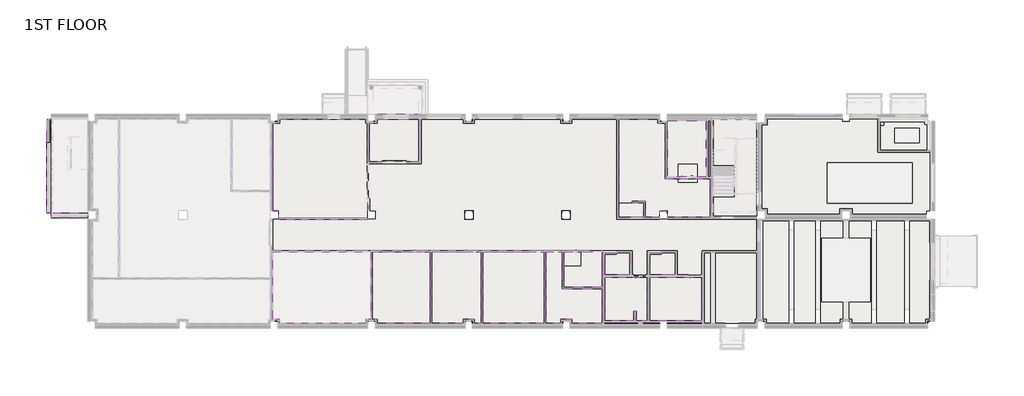
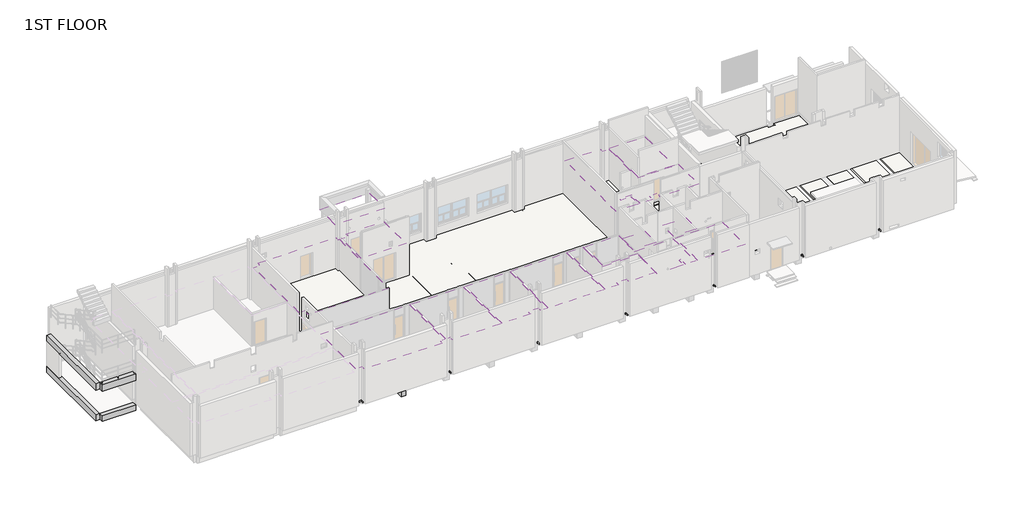
# One storey, part 8 of 15: 26 slabs, 15 coverings, 5 beams.
# Revit data of these elements (continued)
# Type "H_CE_AR_B09_2L Gypsum Board_T Bar_9T_C4" (continued)
#   Layers, outside or top first: 9.5 mm "00_Finish_Gypsum Board" (function 4); 9.5 mm "00_Finish_Gypsum Board" (function 4)
# Type "H_CE_AR_B09_Aluminum Spandrel_M Bar_0.8T_C9"
#   built-in parameter 1002203 = 1 (stored number, unit not read)
#   built-in parameter 1002202 = 1 (stored number, unit not read)
#   Layers, outside or top first: 0.8 mm "00.Ceiling_Aluminum Spandrel" (function 4)
# Type "H_CE_AR_B09_SMC Ceiling_T Bar_300x300x0.8T_C6"
#   built-in parameter 1002203 = 1 (stored number, unit not read)
#   built-in parameter 1002202 = 1 (stored number, unit not read)
#   Layers, outside or top first: 0.8 mm "00.Ceiling_SMC" (function 4)
# Type "H_CE_AR_B09_Souns Absorbing Soft Fiber Board_T Bar_600x600x9T_C5"
#   built-in parameter 1002203 = 1 (stored number, unit not read)
#   built-in parameter 1002202 = 1 (stored number, unit not read)
#   Layers, outside or top first: 9 mm "00.Ceiling_Sound Absorbing Soft Fiber Board" (function 4)
# Type "H_CE_AR_B09_Stainless Hairline Finish_3T"
#   built-in parameter 1002203 = 1 (stored number, unit not read)
#   built-in parameter 1002202 = 1 (stored number, unit not read)
#   Layers, outside or top first: 3 mm "00.Finish_Stainless Hairline" (function 4)
# Type "H_FL_AR_S17_RC Slab_T150_1S1"
#   Keynote = ""
#   Type Comments = "CV-AG"
#   Description = ""
#   H_Rebar Ratio = 0.1
#   Function = 1
#   Layers, outside or top first: 150 mm "Concrete_f'c=28MPa(Cylender)" (function 1)
# Type "H_FL_AR_S17_RC Slab_T150_GS1"
#   Keynote = ""
#   Type Comments = "CV-AG"
#   Description = ""
#   H_Rebar Ratio = 0.1
#   Function = 1
#   Layers, outside or top first: 150 mm "Concrete_f'c=28MPa(Cylender)" (function 1)
# Type "H_FL_AR_S17_RC Slab_T200_SS1"
#   Keynote = ""
#   Type Comments = "CV-AG"
#   Description = ""
#   H_Rebar Ratio = 0.1
#   Function = 1
#   Layers, outside or top first: 200 mm "Concrete_f'c=28MPa(Cylender)" (function 1)
# Type "H_FL_AR_B07_Wood Tile_600x600xT3_F8"
#   Keynote = ""
#   Type Comments = "Finish"
#   Description = ""
#   Function = 1
#   Layers, outside or top first: 3 mm "00_Finish_Wood Tile" (function 4); 27 mm "00_Concrete_Cement Mortar" (function 1)
# Type "H_FL_AR_B07_Deco Tile_600x600xT3"
#   Keynote = ""
#   Type Comments = "Finish"
#   Description = ""
#   Function = 1
#   Layers, outside or top first: 3 mm "00_Finish_Deco Tile" (function 4); 27 mm "00_Concrete_Cement Mortar" (function 1)
# Type "H_FL_AR_B07_Polishing Tile_600x600xT3"
#   Keynote = ""
#   Type Comments = "Finish"
#   Description = ""
#   Function = 1
#   Layers, outside or top first: 3 mm "00_Finish_Polishing Tile" (function 4); 27 mm "00_Concrete_Cement Mortar" (function 1)
# Type "H_FL_AR_B07_Capet Tile_600x600xT3"
#   Keynote = ""
#   Type Comments = "Finish"
#   Description = ""
#   Function = 1
#   Layers, outside or top first: 3 mm "00_Finish_Carpet Tile" (function 4); 27 mm "00_Concrete_Cement Mortar" (function 1)
# Type "H_FL_AR_B07_Wood Tile_600x600xT110_F8"
#   Keynote = ""
#   Type Comments = "Finish"
#   Description = ""
#   Function = 1
#   Layers, outside or top first: 3 mm "00_Finish_Wood Tile" (function 4); 107 mm "00_Concrete_Cement Mortar" (function 1)
# Type "H_FL_AR_B07_Non-Slip Ceramic Tile_L Waterproof_300x300xT4"
#   Keynote = ""
#   Type Comments = "Finish"
#   Description = ""
#   Function = 0
#   Layers, outside or top first: 4 mm "00_Finish_Ceramic Tile" (function 4); 96 mm "00_Concrete_Cement Mortar" (function 1)
# Type "H_FL_AR_B07_Granite Tile_150x150xT30"
#   Keynote = ""
#   Type Comments = "Finish"
#   Description = ""
#   Function = 0
#   Layers, outside or top first: 30 mm "00_Stone_Granite" (function 4); 60 mm "00_Concrete_Cement Mortar" (function 1)
# Type "H_FL_AR_B07_Granite Tile_150x150xT30(Mortar_T170)"
#   Keynote = ""
#   Type Comments = "Finish"
#   Description = ""
#   Function = 0
#   Layers, outside or top first: 30 mm "00_Stone_Granite" (function 4); 170 mm "00_Concrete_Cement Mortar" (function 1)
# Type "H_FL_AR_S17_RC Slab_T300"
#   Keynote = ""
#   Type Comments = "CV-AG"
#   Description = ""
#   H_Rebar Ratio = 0.12
#   Function = 1
#   Layers, outside or top first: 300 mm "Concrete_f'c=28MPa(Cylender)" (function 1)
# Element 1 (IfcBeam, "RC Beam_Rectangular : H_SB_AR S16_TG-UG_450x800_1B1A")
#   Comments = ""
#   hec_material3 = none
#   hec_material2 = none
#   hec_material1 = none
#   Structural Material = Concrete_f'c=28MPa(Cylender)
#   Phase Created = New Construction
#   Materials on its faces: "Concrete_f'c=28MPa(Cylender)"
# Element 2 (IfcBeam, "RC Beam_Rectangular : H_SB_AR S16_RC Beam-AG_400x530_SG1A")
#   Comments = ""
#   hec_material3 = none
#   hec_material2 = none
#   hec_material1 = none
#   Structural Material = Concrete_f'c=28MPa(Cylender)
#   Phase Created = New Construction
#   Materials on its faces: "Concrete_f'c=28MPa(Cylender)"
# Element 3 (IfcBeam, "RC Beam_Rectangular : H_SB_AR S16_RC Beam-AG_400x600_SG2")
#   Comments = ""
#   hec_material3 = none
#   hec_material2 = none
#   hec_material1 = none
#   Structural Material = Concrete_f'c=28MPa(Cylender)
#   Phase Created = New Construction
#   Materials on its faces: "Concrete_f'c=28MPa(Cylender)"
# Element 4 (IfcBeam, "RC Beam_Rectangular : H_SB_AR S16_RC Beam-AG_400x600_SWG2")
#   Comments = ""
#   hec_material3 = none
#   hec_material2 = none
#   hec_material1 = none
#   Structural Material = Concrete_f'c=28MPa(Cylender)
#   Phase Created = New Construction
#   Materials on its faces: "Concrete_f'c=28MPa(Cylender)"
# Element 5 (IfcBeam, "RC Beam_Rectangular : H_SB_AR S16_RC Beam-AG_400x600_SG1")
#   Comments = ""
#   hec_material3 = none
#   hec_material2 = none
#   hec_material1 = none
#   Structural Material = Concrete_f'c=28MPa(Cylender)
#   Phase Created = New Construction
#   Materials on its faces: "Concrete_f'c=28MPa(Cylender)"
# Elements 6, 10, 11, 13 (IfcCovering, "H_CE_AR_B09_2L Gypsum Board_T Bar_9T_C4")
#   Height Offset From Level = 3030 mm
#   Phase Created = New Construction
#   Materials on its faces: "00_Finish_Gypsum Board"
# Element 7 (IfcCovering, "H_CE_AR_B09_Aluminum Spandrel_M Bar_0.8T_C9")
#   Height Offset From Level = 3030 mm
#   Phase Created = New Construction
#   Materials on its faces: "00.Ceiling_Aluminum Spandrel"
# Element 8 (IfcCovering, "H_CE_AR_B09_2L Gypsum Board_T Bar_9T_C4")
#   Height Offset From Level = 3110 mm
#   Phase Created = New Construction
#   Materials on its faces: "00_Finish_Gypsum Board"
# Element 9 (IfcCovering, "H_CE_AR_B09_SMC Ceiling_T Bar_300x300x0.8T_C6")
#   Height Offset From Level = 3000 mm
#   Phase Created = New Construction
#   Materials on its faces: "00.Ceiling_SMC"
# Elements 12, 14, 15 (IfcCovering, "H_CE_AR_B09_Souns Absorbing Soft Fiber Board_T Bar_600x600x9T_C5")
#   Height Offset From Level = 3030 mm
#   Phase Created = New Construction
#   Materials on its faces: "00.Ceiling_Sound Absorbing Soft Fiber Board"
# Elements 16, 17, 18, 19 (IfcCovering, "H_CE_AR_B09_2L Gypsum Board_T Bar_9T_C4")
#   Height Offset From Level = 2700 mm
#   Phase Created = New Construction
#   Materials on its faces: "00_Finish_Gypsum Board"
# Element 20 (IfcCovering, "H_CE_AR_B09_Stainless Hairline Finish_3T")
#   Height Offset From Level = 3900 mm
#   Phase Created = New Construction
#   Materials on its faces: "00.Finish_Stainless Hairline"
# Element 21 (IfcSlab, "H_FL_AR_S17_RC Slab_T150_1S1")
#   Comments = ""
#   TMP_Element Name = "SS2"
#   Height Offset From Level = 0 mm
#   built-in parameter 1001954 = 1
#   Phase Created = New Construction
#   Materials on its faces: "Concrete_f'c=28MPa(Cylender)"
# Element 22 (IfcSlab, "H_FL_AR_S17_RC Slab_T150_1S1")
#   Comments = ""
#   TMP_Element Name = "SS2"
#   Height Offset From Level = -100 mm
#   built-in parameter 1001954 = 1
#   Phase Created = New Construction
#   Materials on its faces: "Concrete_f'c=28MPa(Cylender)"
# Element 23 (IfcSlab, "H_FL_AR_S17_RC Slab_T150_GS1")
#   Comments = ""
#   TMP_Element Name = "SS2"
#   built-in parameter 1001955 = 3.14159 (stored number, unit not read)
#   Height Offset From Level = 0 mm
#   built-in parameter 1001954 = 1
#   Phase Created = New Construction
#   Materials on its faces: "Concrete_f'c=28MPa(Cylender)"
# Element 24 (IfcSlab, "H_FL_AR_S17_RC Slab_T150_1S1")
#   Comments = ""
#   TMP_Element Name = "SS2"
#   built-in parameter 1001955 = 3.14159 (stored number, unit not read)
#   Height Offset From Level = -100 mm
#   built-in parameter 1001954 = 1
#   Phase Created = New Construction
#   Materials on its faces: "Concrete_f'c=28MPa(Cylender)"
# Element 25 (IfcSlab, "H_FL_AR_S17_RC Slab_T200_SS1")
#   Comments = ""
#   TMP_Element Name = "SS2"
#   Height Offset From Level = 0 mm
#   built-in parameter 1001954 = 1
#   Phase Created = New Construction
#   Materials on its faces: "Concrete_f'c=28MPa(Cylender)"
# Element 26 (IfcSlab, "H_FL_AR_S17_RC Slab_T150_GS1")
#   Comments = ""
#   TMP_Element Name = "SS2"
#   Height Offset From Level = 0 mm
#   built-in parameter 1001954 = 1
#   Phase Created = New Construction
#   Materials on its faces: "Concrete_f'c=28MPa(Cylender)"
# Elements 27, 43 (IfcSlab, "H_FL_AR_B07_Wood Tile_600x600xT3_F8")
#   Height Offset From Level = 30 mm
#   Phase Created = New Construction
#   Materials on its faces: "00_Concrete_Cement Mortar", "00_Finish_Wood Tile"
# Elements 28, 31, 40, 42 (IfcSlab, "H_FL_AR_B07_Deco Tile_600x600xT3")
#   Height Offset From Level = 30 mm
#   Phase Created = New Construction
#   Materials on its faces: "00_Concrete_Cement Mortar", "00_Finish_Deco Tile"
# Element 29 (IfcSlab, "H_FL_AR_B07_Polishing Tile_600x600xT3")
#   built-in parameter 1001955 = 1.5708 (stored number, unit not read)
#   Height Offset From Level = 30 mm
#   Phase Created = New Construction
#   Materials on its faces: "00_Concrete_Cement Mortar", "00_Finish_Polishing Tile"
# Element 30 (IfcSlab, "H_FL_AR_B07_Wood Tile_600x600xT3_F8")
#   built-in parameter 1001955 = 1.5708 (stored number, unit not read)
#   Height Offset From Level = 30 mm
#   Phase Created = New Construction
#   Materials on its faces: "00_Concrete_Cement Mortar", "00_Finish_Wood Tile"
# Element 32 (IfcSlab, "H_FL_AR_B07_Capet Tile_600x600xT3")
#   Height Offset From Level = 30 mm
#   Phase Created = New Construction
#   Materials on its faces: "00_Concrete_Cement Mortar", "00_Finish_Carpet Tile"
# Element 33 (IfcSlab, "H_FL_AR_B07_Deco Tile_600x600xT3")
#   built-in parameter 1001955 = 1.5708 (stored number, unit not read)
#   Height Offset From Level = 30 mm
#   Phase Created = New Construction
#   Materials on its faces: "00_Concrete_Cement Mortar", "00_Finish_Deco Tile"
# Element 34 (IfcSlab, "H_FL_AR_B07_Wood Tile_600x600xT110_F8")
#   Height Offset From Level = 110 mm
#   Phase Created = New Construction
#   Materials on its faces: "00_Concrete_Cement Mortar", "00_Finish_Wood Tile"
# Elements 35, 36, 37, 38, 41 (IfcSlab, "H_FL_AR_B07_Non-Slip Ceramic Tile_L Waterproof_300x300xT4")
#   Height Offset From Level = 0 mm
#   Phase Created = New Construction
#   Materials on its faces: "00_Concrete_Cement Mortar", "00_Finish_Ceramic Tile"
# Element 39 (IfcSlab, "H_FL_AR_B07_Wood Tile_600x600xT110_F8")
#   built-in parameter 1001955 = 1.5708 (stored number, unit not read)
#   Height Offset From Level = 110 mm
#   Phase Created = New Construction
#   Materials on its faces: "00_Concrete_Cement Mortar", "00_Finish_Wood Tile"
# Element 44 (IfcSlab, "H_FL_AR_B07_Granite Tile_150x150xT30")
#   Height Offset From Level = 200 mm
#   Phase Created = New Construction
#   Materials on its faces: "00_Concrete_Cement Mortar", "00_Stone_Granite"
# Element 45 (IfcSlab, "H_FL_AR_B07_Granite Tile_150x150xT30(Mortar_T170)")
#   Height Offset From Level = 200 mm
#   Phase Created = New Construction
#   Materials on its faces: "00_Concrete_Cement Mortar", "00_Stone_Granite"
# Element 46 (IfcSlab, "H_FL_AR_S17_RC Slab_T300")
#   Comments = ""
#   TMP_Element Name = "SS2"
#   Height Offset From Level = -150 mm
#   built-in parameter 1001954 = 1
#   Phase Created = New Construction
#   Materials on its faces: "Concrete_f'c=28MPa(Cylender)"
# Materials
#   "00_Finish_Gypsum Board": class "Finish", colour RGB 171 170 168, transparency 0, Description = "Gypsum Board", Cost = 0, Image = Finishes.Gypsum Board.Painted.White.jpg
#   "00.Ceiling_Aluminum Spandrel": class "Generic", colour RGB 253 254 255, transparency 0, Description = "Acoustic ceiling tile", Cost = 0
#   "00.Ceiling_SMC": class "Generic", colour RGB 237 237 236, transparency 0, Description = "Acoustic ceiling tile", Cost = 0
#   "00.Ceiling_Sound Absorbing Soft Fiber Board": class "Generic", colour RGB 237 237 236, transparency 0, Description = "Acoustic ceiling tile", Cost = 0
#   "00.Finish_Stainless Hairline": class "Generic", colour RGB 149 149 149, transparency 0, Description = "Acoustic ceiling tile", Cost = 0
#   "Concrete_f'c=28MPa(Cylender)": class "Concrete", colour RGB 176 176 176, transparency 0, Description = "Reinf. Conc.", Cost = 0, Image = Concrete.Cast-In-Place.Flat.Polished.Grey.jpg
#   "00_Finish_Wood Tile": class "Finish", colour RGB 233 219 207, transparency 0, Description = "Ceramic Tile", Cost = 0
#   "00_Concrete_Cement Mortar": class "Concrete", colour RGB 183 186 184, transparency 0, Description = "Cement Mortar", Cost = 0, Image = Concrete.Cast-In-Place.Flat.Broom.Grey.jpg
#   "00_Finish_Deco Tile": class "Finish", colour RGB 245 245 245, transparency 0, Description = "Ceramic Tile", Cost = 0
#   "00_Finish_Polishing Tile": class "Finish", colour RGB 245 245 245, transparency 0, Description = "Ceramic Tile", Cost = 0
#   "00_Finish_Carpet Tile": class "Finish", colour RGB 68 67 66, transparency 0, Description = "Carpet", Cost = 0
#   "00_Finish_Ceramic Tile": class "Finish", colour RGB 245 245 245, transparency 0, Description = "Ceramic Tile", Cost = 0, Image = none
#   "00_Stone_Granite": class "Stone", colour RGB 99 103 98, transparency 0, Description = "Granite", Cost = 0, Image = Masonry.Stone.Granite.Square.Stacked.Polished.Black-White.jpg
# Room at (66747.5, -1477.5) mm, phase "New Construction", upper level "1ST FLOOR", upper offset 5800 mm, lower offset 0 mm
#   Comments = ""
#   Occupancy = "1"
#   Number = "124"
#   Name = "F.O TANK ROOM"
#   H_Room H or CH = 5.8 mm
# Room at (48912.5, -2537.5) mm, phase "New Construction", upper level "1ST FLOOR", upper offset 5800 mm, lower offset 0 mm
#   Comments = ""
#   Occupancy = "1"
#   Number = "109"
#   Name = "SHOWER ROOM"
#   H_Room H or CH = 3 mm
# Room at (61920.25, -12686.25) mm, phase "New Construction", upper level "1ST FLOOR", upper offset 5800 mm, lower offset 0 mm
#   Comments = ""
#   Occupancy = "1"
#   Number = "125"
#   Name = "HVAC ROOM"
#   H_Room H or CH = 5.8 mm
# Room at (24871.5, -1826.5) mm, phase "New Construction", upper level "1ST FLOOR", upper offset 5800 mm, lower offset 0 mm
#   Comments = ""
#   Occupancy = "1"
#   Number = "105"
#   Name = "AIR LOCK"
#   H_Room H or CH = 3 mm
# Room at (52496.5, -14023.5) mm, phase "New Construction", upper level "1ST FLOOR", upper offset 5800 mm, lower offset 0 mm
#   Comments = ""
#   Occupancy = "1"
#   Number = "122"
#   Name = "CYLINDER ROOM"
#   H_Room H or CH = 3 mm
# Room at (43200, -12000) mm, phase "New Construction", upper level "1ST FLOOR", upper offset 5800 mm, lower offset 0 mm
#   Comments = ""
#   Occupancy = "1"
#   Number = "118"
#   Name = "DISABLED TOLET(M)"
#   H_Room H or CH = 2.7 mm
# Room at (43900, -14887.5) mm, phase "New Construction", upper level "1ST FLOOR", upper offset 5800 mm, lower offset 0 mm
#   Comments = ""
#   Occupancy = "1"
#   Number = "120"
#   Name = "TOILET(M)"
#   H_Room H or CH = 2.7 mm
# Room at (46900, -12000) mm, phase "New Construction", upper level "1ST FLOOR", upper offset 5800 mm, lower offset 0 mm
#   Comments = ""
#   Occupancy = "1"
#   Number = "119"
#   Name = "DISABLED TOILET(W)"
#   H_Room H or CH = 2.7 mm
# Room at (48000, -14887.5) mm, phase "New Construction", upper level "1ST FLOOR", upper offset 5800 mm, lower offset 0 mm
#   Comments = ""
#   Occupancy = "1"
#   Number = "121"
#   Name = "TOILET(W)"
#   H_Room H or CH = 2.7 mm
# Room at (47084, -5635.02) mm, phase "New Construction", upper level "1ST FLOOR", upper offset 5800 mm, lower offset 0 mm
#   Comments = ""
#   Occupancy = "1"
#   Number = "108"
#   Name = "LOCKER ROOM"
#   H_Room H or CH = 3 mm
# Room at (34768, -8500) mm, phase "New Construction", upper level "1ST FLOOR", upper offset 5800 mm, lower offset 0 mm
#   Comments = ""
#   Occupancy = "1"
#   Number = "111"
#   Name = "CORRIDOR"
#   H_Room H or CH = 5.8 mm
# Room at (52862.5, -4131) mm, phase "New Construction", upper level "1ST FLOOR", upper offset 5800 mm, lower offset 0 mm
#   Comments = ""
#   Occupancy = "1"
#   Number = "110"
#   Name = "STAIRCASE"
#   H_Room H or CH = 5.8 mm
# Room at (62081, -3919) mm, phase "New Construction", upper level "1ST FLOOR", upper offset 9300 mm, lower offset 0 mm
#   Comments = ""
#   Number = "123"
#   Name = "EDG ROOM"
#   H_Room H or CH = 9.2 mm
# Room at (44419.201, -7539.972) mm, phase "New Construction", upper level "1ST FLOOR", upper offset 5800 mm, lower offset 0 mm
#   Comments = ""
#   Occupancy = "1"
#   Number = "151"
#   Name = "LOCKER ENTRANCE"
#   H_Room H or CH = 3 mm
# Room at (33678.344, -3773.505) mm, phase "New Construction", upper level "1ST FLOOR", upper offset 5800 mm, lower offset 0 mm
#   Comments = ""
#   Occupancy = "1"
#   Number = "107"
#   Name = "OFFICE ROOM"
#   H_Room H or CH = 5.8 mm
# Room at (40496.214, -12367.394) mm, phase "New Construction", upper level "1ST FLOOR", upper offset 5800 mm, lower offset 0 mm
#   Comments = ""
#   Occupancy = "1"
#   Number = "116"
#   Name = "MAMA'S REST ROOM"
#   H_Room H or CH = 3 mm
# Room at (39361.919, -14919.559) mm, phase "New Construction", upper level "1ST FLOOR", upper offset 5800 mm, lower offset 0 mm
#   Comments = ""
#   Occupancy = "1"
#   Number = "117"
#   Name = "STORAGE"
#   H_Room H or CH = 3 mm
# Room at (34862.546, -13898.693) mm, phase "New Construction", upper level "1ST FLOOR", upper offset 5800 mm, lower offset 0 mm
#   Comments = ""
#   Occupancy = "1"
#   Number = "115"
#   Name = "PRESIDENT ROOM"
#   H_Room H or CH = 3 mm
# Room at (30211.935, -13917.598) mm, phase "New Construction", upper level "1ST FLOOR", upper offset 5800 mm, lower offset 0 mm
#   Comments = ""
#   Occupancy = "1"
#   Number = "114"
#   Name = "PARTNER'S OFFICE"
#   H_Room H or CH = 3 mm
# Room at (25315.559, -14049.933) mm, phase "New Construction", upper level "1ST FLOOR", upper offset 5800 mm, lower offset 0 mm
#   Comments = ""
#   Occupancy = "1"
#   Number = "113"
#   Name = "REST ROOM"
#   H_Room H or CH = 3 mm
# Room at (19265.983, -13936.503) mm, phase "New Construction", upper level "1ST FLOOR", upper offset 5800 mm, lower offset 0 mm
#   Comments = ""
#   Occupancy = "1"
#   Number = "112"
#   Name = "CONFERENCE ROOM"
#   H_Room H or CH = 3 mm
# Room at (18995.787, -4264.529) mm, phase "New Construction", upper level "1ST FLOOR", upper offset 5800 mm, lower offset 0 mm
#   Comments = ""
#   Occupancy = "1"
#   Number = "104"
#   Name = "CANTEEN"
#   H_Room H or CH = 3 mm
# Room at (12951.563, -3235.471) mm, phase "New Construction", upper level "1ST FLOOR", upper offset 5800 mm, lower offset 0 mm
#   Comments = ""
#   Occupancy = "1"
#   Number = "102"
#   Name = "MEETING ROOM"
#   H_Room H or CH = 3 mm
# Room at (8524.954, -7021.7) mm, phase "New Construction", upper level "1ST FLOOR", upper offset 5800 mm, lower offset 0 mm
#   Comments = ""
#   Occupancy = "1"
#   Number = "101"
#   Name = "CENTRAL CONTROL ROOM"
#   H_Room H or CH = 3 mm
# Room at (1443.913, -5932.309) mm, phase "New Construction", upper level "1ST FLOOR", upper offset 5800 mm, lower offset 0 mm
#   Comments = ""
#   Occupancy = "1"
#   Number = "152"
#   Name = "CCR SIDE"
#   H_Room H or CH = 3 mm
# Room at (5610.834, -15410.011) mm, phase "New Construction", upper level "1ST FLOOR", upper offset 5800 mm, lower offset 0 mm
#   Comments = ""
#   Occupancy = "1"
#   Number = "103"
#   Name = "ENGINEERING ROOM"
#   H_Room H or CH = 3 mm
